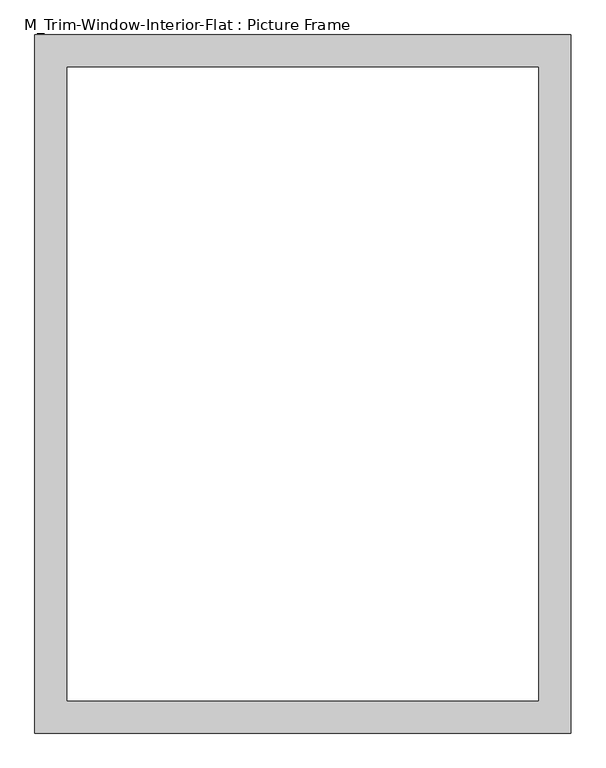
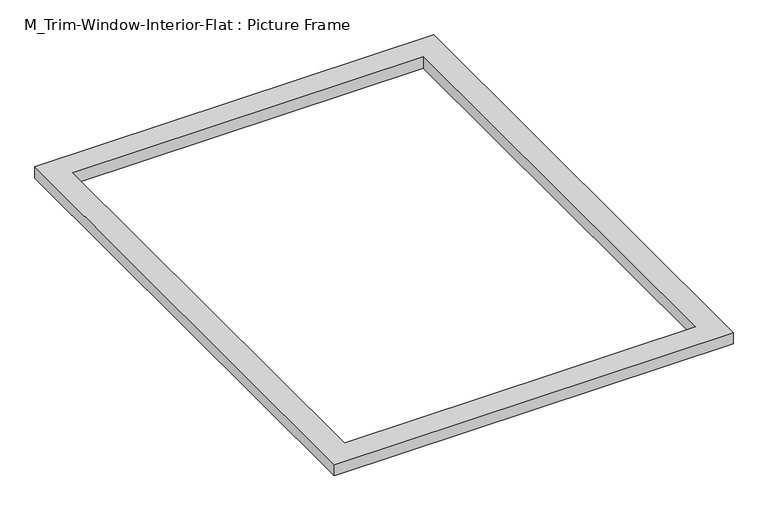
"""IFC4 building model written with IfcOpenShell, lengths in millimetres: proxy geometry, M_Trim-Window-Interior-Flat : Picture Frame."""

from ifc_helpers import new_model, si_unit, origin, origin_with_axes, place, context, project, spatial, polyline, outline, extrude, source, transform, mapped, element, save


def m_trim_window_interior_flat_picture_frame_24fe8ef8(model_context):
    return source(origin(), model_context, "Body", "SweptSolid", [
        extrude(outline(polyline([(497.3, 47.3), (497.3, -1247.3), (-497.3, -1247.3), (-497.3, 47.3), (497.3, 47.3)]), holes=[polyline([(437.3, -12.7), (-437.3, -12.7), (-437.3, -1187.3), (437.3, -1187.3), (437.3, -12.7)])]), origin_with_axes(), (0.0, 0.0, 1.0), 30.0),
    ])


if __name__ == "__main__":
    model = new_model("IFC4")
    model_context = context("Model", 3, world=origin())
    ifc_project = project(units=[si_unit("LENGTHUNIT", "METRE", prefix="MILLI")], contexts=[model_context])
    site = spatial("IfcSite", under=ifc_project)
    building = spatial("IfcBuilding", under=site)
    placement = place(None, origin())
    m_trim_window_interior_flat_picture_frame_shape = m_trim_window_interior_flat_picture_frame_24fe8ef8(model_context)
    element("IfcBuildingElementProxy", 1, Name="M_Trim-Window-Interior-Flat : Picture Frame", ObjectType="M_Trim-Window-Interior-Flat : Picture Frame", at=placement, inside=building, context=model_context, shape_type="MappedRepresentation", body=[
        mapped(m_trim_window_interior_flat_picture_frame_shape, transform((0.0, 0.0, 0.0), x_axis=(1.0, 0.0, 0.0), y_axis=(0.0, 1.0, 0.0), z_axis=(0.0, 0.0, 1.0))),
    ])
    save(model, "model.ifc")

# Revit data of these elements
# Type "M_Trim-Window-Interior-Flat : Picture Frame"
#   Trim Thickness_Picture Frame = 30 mm
#   Trim Width = 60 mm
#   Trim Thickness_with Sill = 20 mm
#   Sill Thickness = 30 mm
#   Opening Width [instance default] = 600 mm
#   Opening Height [instance default] = 900 mm
#   Default Elevation = 1200 mm
#   Sill = no
#   Picture Frame = yes
#   Trim Material [instance default] = none
# Element 1 (IfcBuildingElementProxy, "M_Trim-Window-Interior-Flat : Picture Frame")
#   Opening Width = 900 mm
#   Opening Height = 1200 mm
#   Trim Material = Wood - Stained
#   Materials on its faces: "Wood - Stained"
# Materials
#   "Wood - Stained": class "Wood", colour RGB 173 132 96, transparency 0, Cost = 0
